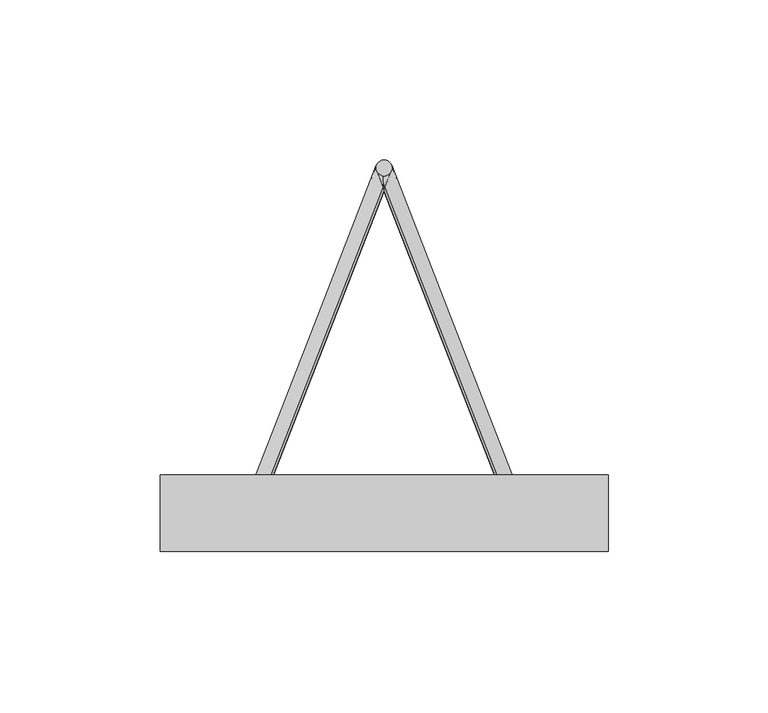
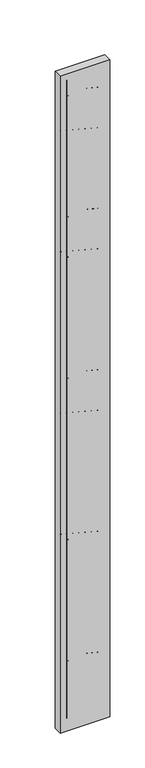
"""IFC4 building model written with IfcOpenShell, lengths in millimetres: proxy geometry, Vigota 1 (Pano 8) (Mf = 193)."""

from ifc_helpers import new_model, si_unit, point, frame, frame_2d, origin, origin_with_axes, origin_2d, place, context, project, spatial, polyline, circle_curve, trimmed, segment, composite_curve, outline, extrude, source, transform, mapped, element, save


def structural_framing_4a41f4d1(model_context):
    return source(origin(), model_context, "Body", "SweptSolid", [
        extrude(outline(polyline([(-70.0, 12.0), (70.0, 12.0), (70.0, -12.0), (-70.0, -12.0), (-70.0, 12.0)])), origin_with_axes(), (0.0, 0.0, 1.0), 1952.601886),
        extrude(outline(composite_curve([segment(trimmed(circle_curve(frame_2d((42.0, 0.0)), 2.5), [point((44.5, 0.0))], [point((39.5, 0.0))], False, "CARTESIAN"), True, "CONTINUOUS"), segment(trimmed(circle_curve(frame_2d((42.0, 0.0)), 2.5), [point((39.5, 0.0))], [point((44.5, 0.0))], False, "CARTESIAN"), True, "CONTINUOUS")], self_intersect=False)), frame((0.0, 0.0, 28.0), z_axis=(0.0, 0.0, 1.0), x_axis=(1.0, 0.0, 0.0)), (0.0, 0.0, 1.0), 1896.601886),
        extrude(outline(composite_curve([segment(trimmed(circle_curve(frame_2d((0.0, 108.0)), 2.5), [point((2.5, 108.0))], [point((-2.5, 108.0))], False, "CARTESIAN"), True, "CONTINUOUS"), segment(trimmed(circle_curve(frame_2d((0.0, 108.0)), 2.5), [point((-2.5, 108.0))], [point((2.5, 108.0))], False, "CARTESIAN"), True, "CONTINUOUS")], self_intersect=False)), frame((0.0, 0.0, 86.300943), z_axis=(0.0, 0.0, 1.0), x_axis=(1.0, 0.0, 0.0)), (0.0, 0.0, 1.0), 1780.0),
        extrude(outline(composite_curve([segment(trimmed(circle_curve(origin_2d(), 2.5), [point((2.5, 0.0))], [point((-2.5, 0.0))], False, "CARTESIAN"), True, "CONTINUOUS"), segment(trimmed(circle_curve(origin_2d(), 2.5), [point((-2.5, 0.0))], [point((2.5, 0.0))], False, "CARTESIAN"), True, "CONTINUOUS")], self_intersect=False)), frame((42.0, 0.0, 76.300943), z_axis=(-0.3218603428886276, 0.8276408817707567, 0.4598004898837537), x_axis=(0.8192319205108605, -3.936835275445103e-11, 0.5734623443750141)), (0.0, 0.0, 1.0), 130.491379),
        extrude(outline(composite_curve([segment(trimmed(circle_curve(origin_2d(), 2.5), [point((2.5, 0.0))], [point((-2.5, 0.0))], False, "CARTESIAN"), True, "CONTINUOUS"), segment(trimmed(circle_curve(origin_2d(), 2.5), [point((-2.5, 0.0))], [point((2.5, 0.0))], False, "CARTESIAN"), True, "CONTINUOUS")], self_intersect=False)), frame((0.0, 108.0, 136.300943), z_axis=(0.3218603428886276, -0.8276408817707567, 0.4598004898837537), x_axis=(0.8192319205108605, -3.936835275445103e-11, -0.5734623443750141)), (0.0, 0.0, 1.0), 130.491379),
        extrude(outline(composite_curve([segment(trimmed(circle_curve(origin_2d(), 2.5), [point((2.5, 0.0))], [point((-2.5, 0.0))], False, "CARTESIAN"), True, "CONTINUOUS"), segment(trimmed(circle_curve(origin_2d(), 2.5), [point((-2.5, 0.0))], [point((2.5, 0.0))], False, "CARTESIAN"), True, "CONTINUOUS")], self_intersect=False)), frame((42.0, 0.0, 196.300943), z_axis=(-0.3218603428886276, 0.8276408817707567, 0.4598004898837537), x_axis=(0.8192319205108605, -3.936835275445103e-11, 0.5734623443750141)), (0.0, 0.0, 1.0), 130.491379),
        extrude(outline(composite_curve([segment(trimmed(circle_curve(origin_2d(), 2.5), [point((2.5, 0.0))], [point((-2.5, 0.0))], False, "CARTESIAN"), True, "CONTINUOUS"), segment(trimmed(circle_curve(origin_2d(), 2.5), [point((-2.5, 0.0))], [point((2.5, 0.0))], False, "CARTESIAN"), True, "CONTINUOUS")], self_intersect=False)), frame((0.0, 108.0, 256.300943), z_axis=(0.3218603428886276, -0.8276408817707567, 0.4598004898837537), x_axis=(0.8192319205108605, -3.936835275445103e-11, -0.5734623443750141)), (0.0, 0.0, 1.0), 130.491379),
        extrude(outline(composite_curve([segment(trimmed(circle_curve(origin_2d(), 2.5), [point((2.5, 0.0))], [point((-2.5, 0.0))], False, "CARTESIAN"), True, "CONTINUOUS"), segment(trimmed(circle_curve(origin_2d(), 2.5), [point((-2.5, 0.0))], [point((2.5, 0.0))], False, "CARTESIAN"), True, "CONTINUOUS")], self_intersect=False)), frame((42.0, 0.0, 316.300943), z_axis=(-0.3218603428886276, 0.8276408817707567, 0.4598004898837537), x_axis=(0.8192319205108605, -3.936835275445103e-11, 0.5734623443750141)), (0.0, 0.0, 1.0), 130.491379),
        extrude(outline(composite_curve([segment(trimmed(circle_curve(origin_2d(), 2.5), [point((2.5, 0.0))], [point((-2.5, 0.0))], False, "CARTESIAN"), True, "CONTINUOUS"), segment(trimmed(circle_curve(origin_2d(), 2.5), [point((-2.5, 0.0))], [point((2.5, 0.0))], False, "CARTESIAN"), True, "CONTINUOUS")], self_intersect=False)), frame((0.0, 108.0, 376.300943), z_axis=(0.3218603428886276, -0.8276408817707567, 0.4598004898837537), x_axis=(0.8192319205108605, -3.936835275445103e-11, -0.5734623443750141)), (0.0, 0.0, 1.0), 130.491379),
        extrude(outline(composite_curve([segment(trimmed(circle_curve(origin_2d(), 2.5), [point((2.5, 0.0))], [point((-2.5, 0.0))], False, "CARTESIAN"), True, "CONTINUOUS"), segment(trimmed(circle_curve(origin_2d(), 2.5), [point((-2.5, 0.0))], [point((2.5, 0.0))], False, "CARTESIAN"), True, "CONTINUOUS")], self_intersect=False)), frame((42.0, 0.0, 436.300943), z_axis=(-0.3218603428886276, 0.8276408817707567, 0.4598004898837537), x_axis=(0.8192319205108605, -3.936835275445103e-11, 0.5734623443750141)), (0.0, 0.0, 1.0), 130.491379),
        extrude(outline(composite_curve([segment(trimmed(circle_curve(origin_2d(), 2.5), [point((2.5, 0.0))], [point((-2.5, 0.0))], False, "CARTESIAN"), True, "CONTINUOUS"), segment(trimmed(circle_curve(origin_2d(), 2.5), [point((-2.5, 0.0))], [point((2.5, 0.0))], False, "CARTESIAN"), True, "CONTINUOUS")], self_intersect=False)), frame((0.0, 108.0, 496.300943), z_axis=(0.3218603428886276, -0.8276408817707567, 0.4598004898837537), x_axis=(0.8192319205108605, -3.936835275445103e-11, -0.5734623443750141)), (0.0, 0.0, 1.0), 130.491379),
        extrude(outline(composite_curve([segment(trimmed(circle_curve(origin_2d(), 2.5), [point((2.5, 0.0))], [point((-2.5, 0.0))], False, "CARTESIAN"), True, "CONTINUOUS"), segment(trimmed(circle_curve(origin_2d(), 2.5), [point((-2.5, 0.0))], [point((2.5, 0.0))], False, "CARTESIAN"), True, "CONTINUOUS")], self_intersect=False)), frame((42.0, 0.0, 556.300943), z_axis=(-0.3218603428886276, 0.8276408817707567, 0.4598004898837537), x_axis=(0.8192319205108605, -3.936835275445103e-11, 0.5734623443750141)), (0.0, 0.0, 1.0), 130.491379),
        extrude(outline(composite_curve([segment(trimmed(circle_curve(origin_2d(), 2.5), [point((2.5, 0.0))], [point((-2.5, 0.0))], False, "CARTESIAN"), True, "CONTINUOUS"), segment(trimmed(circle_curve(origin_2d(), 2.5), [point((-2.5, 0.0))], [point((2.5, 0.0))], False, "CARTESIAN"), True, "CONTINUOUS")], self_intersect=False)), frame((0.0, 108.0, 616.300943), z_axis=(0.3218603428886276, -0.8276408817707567, 0.4598004898837537), x_axis=(0.8192319205108605, -3.936835275445103e-11, -0.5734623443750141)), (0.0, 0.0, 1.0), 130.491379),
        extrude(outline(composite_curve([segment(trimmed(circle_curve(origin_2d(), 2.5), [point((2.5, 0.0))], [point((-2.5, 0.0))], False, "CARTESIAN"), True, "CONTINUOUS"), segment(trimmed(circle_curve(origin_2d(), 2.5), [point((-2.5, 0.0))], [point((2.5, 0.0))], False, "CARTESIAN"), True, "CONTINUOUS")], self_intersect=False)), frame((42.0, 0.0, 676.300943), z_axis=(-0.3218603428886276, 0.8276408817707567, 0.4598004898837537), x_axis=(0.8192319205108605, -3.936835275445103e-11, 0.5734623443750141)), (0.0, 0.0, 1.0), 130.491379),
        extrude(outline(composite_curve([segment(trimmed(circle_curve(origin_2d(), 2.5), [point((2.5, 0.0))], [point((-2.5, 0.0))], False, "CARTESIAN"), True, "CONTINUOUS"), segment(trimmed(circle_curve(origin_2d(), 2.5), [point((-2.5, 0.0))], [point((2.5, 0.0))], False, "CARTESIAN"), True, "CONTINUOUS")], self_intersect=False)), frame((0.0, 108.0, 736.300943), z_axis=(0.3218603428886276, -0.8276408817707567, 0.4598004898837537), x_axis=(0.8192319205108605, -3.936835275445103e-11, -0.5734623443750141)), (0.0, 0.0, 1.0), 130.491379),
        extrude(outline(composite_curve([segment(trimmed(circle_curve(origin_2d(), 2.5), [point((2.5, 0.0))], [point((-2.5, 0.0))], False, "CARTESIAN"), True, "CONTINUOUS"), segment(trimmed(circle_curve(origin_2d(), 2.5), [point((-2.5, 0.0))], [point((2.5, 0.0))], False, "CARTESIAN"), True, "CONTINUOUS")], self_intersect=False)), frame((42.0, 0.0, 796.300943), z_axis=(-0.3218603428886276, 0.8276408817707567, 0.4598004898837537), x_axis=(0.8192319205108605, -3.936835275445103e-11, 0.5734623443750141)), (0.0, 0.0, 1.0), 130.491379),
        extrude(outline(composite_curve([segment(trimmed(circle_curve(origin_2d(), 2.5), [point((2.5, 0.0))], [point((-2.5, 0.0))], False, "CARTESIAN"), True, "CONTINUOUS"), segment(trimmed(circle_curve(origin_2d(), 2.5), [point((-2.5, 0.0))], [point((2.5, 0.0))], False, "CARTESIAN"), True, "CONTINUOUS")], self_intersect=False)), frame((0.0, 108.0, 856.300943), z_axis=(0.3218603428886276, -0.8276408817707567, 0.4598004898837537), x_axis=(0.8192319205108605, -3.936835275445103e-11, -0.5734623443750141)), (0.0, 0.0, 1.0), 130.491379),
        extrude(outline(composite_curve([segment(trimmed(circle_curve(origin_2d(), 2.5), [point((2.5, 0.0))], [point((-2.5, 0.0))], False, "CARTESIAN"), True, "CONTINUOUS"), segment(trimmed(circle_curve(origin_2d(), 2.5), [point((-2.5, 0.0))], [point((2.5, 0.0))], False, "CARTESIAN"), True, "CONTINUOUS")], self_intersect=False)), frame((42.0, 0.0, 916.300943), z_axis=(-0.3218603428886276, 0.8276408817707567, 0.4598004898837537), x_axis=(0.8192319205108605, -3.936835275445103e-11, 0.5734623443750141)), (0.0, 0.0, 1.0), 130.491379),
        extrude(outline(composite_curve([segment(trimmed(circle_curve(origin_2d(), 2.5), [point((2.5, 0.0))], [point((-2.5, 0.0))], False, "CARTESIAN"), True, "CONTINUOUS"), segment(trimmed(circle_curve(origin_2d(), 2.5), [point((-2.5, 0.0))], [point((2.5, 0.0))], False, "CARTESIAN"), True, "CONTINUOUS")], self_intersect=False)), frame((0.0, 108.0, 976.300943), z_axis=(0.3218603428886276, -0.8276408817707567, 0.4598004898837537), x_axis=(0.8192319205108605, -3.936835275445103e-11, -0.5734623443750141)), (0.0, 0.0, 1.0), 130.491379),
        extrude(outline(composite_curve([segment(trimmed(circle_curve(origin_2d(), 2.5), [point((2.5, 0.0))], [point((-2.5, 0.0))], False, "CARTESIAN"), True, "CONTINUOUS"), segment(trimmed(circle_curve(origin_2d(), 2.5), [point((-2.5, 0.0))], [point((2.5, 0.0))], False, "CARTESIAN"), True, "CONTINUOUS")], self_intersect=False)), frame((42.0, 0.0, 1036.300943), z_axis=(-0.3218603428886276, 0.8276408817707567, 0.4598004898837537), x_axis=(0.8192319205108605, -3.936835275445103e-11, 0.5734623443750141)), (0.0, 0.0, 1.0), 130.491379),
        extrude(outline(composite_curve([segment(trimmed(circle_curve(origin_2d(), 2.5), [point((2.5, 0.0))], [point((-2.5, 0.0))], False, "CARTESIAN"), True, "CONTINUOUS"), segment(trimmed(circle_curve(origin_2d(), 2.5), [point((-2.5, 0.0))], [point((2.5, 0.0))], False, "CARTESIAN"), True, "CONTINUOUS")], self_intersect=False)), frame((0.0, 108.0, 1096.300943), z_axis=(0.3218603428886276, -0.8276408817707567, 0.4598004898837537), x_axis=(0.8192319205108605, -3.936835275445103e-11, -0.5734623443750141)), (0.0, 0.0, 1.0), 130.491379),
        extrude(outline(composite_curve([segment(trimmed(circle_curve(origin_2d(), 2.5), [point((2.5, 0.0))], [point((-2.5, 0.0))], False, "CARTESIAN"), True, "CONTINUOUS"), segment(trimmed(circle_curve(origin_2d(), 2.5), [point((-2.5, 0.0))], [point((2.5, 0.0))], False, "CARTESIAN"), True, "CONTINUOUS")], self_intersect=False)), frame((42.0, 0.0, 1156.300943), z_axis=(-0.3218603428886276, 0.8276408817707567, 0.4598004898837537), x_axis=(0.8192319205108605, -3.936835275445103e-11, 0.5734623443750141)), (0.0, 0.0, 1.0), 130.491379),
        extrude(outline(composite_curve([segment(trimmed(circle_curve(origin_2d(), 2.5), [point((2.5, 0.0))], [point((-2.5, 0.0))], False, "CARTESIAN"), True, "CONTINUOUS"), segment(trimmed(circle_curve(origin_2d(), 2.5), [point((-2.5, 0.0))], [point((2.5, 0.0))], False, "CARTESIAN"), True, "CONTINUOUS")], self_intersect=False)), frame((0.0, 108.0, 1216.300943), z_axis=(0.3218603428886276, -0.8276408817707567, 0.4598004898837537), x_axis=(0.8192319205108605, -3.936835275445103e-11, -0.5734623443750141)), (0.0, 0.0, 1.0), 130.491379),
        extrude(outline(composite_curve([segment(trimmed(circle_curve(origin_2d(), 2.5), [point((2.5, 0.0))], [point((-2.5, 0.0))], False, "CARTESIAN"), True, "CONTINUOUS"), segment(trimmed(circle_curve(origin_2d(), 2.5), [point((-2.5, 0.0))], [point((2.5, 0.0))], False, "CARTESIAN"), True, "CONTINUOUS")], self_intersect=False)), frame((42.0, 0.0, 1276.300943), z_axis=(-0.3218603428886276, 0.8276408817707567, 0.4598004898837537), x_axis=(0.8192319205108605, -3.936835275445103e-11, 0.5734623443750141)), (0.0, 0.0, 1.0), 130.491379),
        extrude(outline(composite_curve([segment(trimmed(circle_curve(origin_2d(), 2.5), [point((2.5, 0.0))], [point((-2.5, 0.0))], False, "CARTESIAN"), True, "CONTINUOUS"), segment(trimmed(circle_curve(origin_2d(), 2.5), [point((-2.5, 0.0))], [point((2.5, 0.0))], False, "CARTESIAN"), True, "CONTINUOUS")], self_intersect=False)), frame((0.0, 108.0, 1336.300943), z_axis=(0.3218603428886276, -0.8276408817707567, 0.4598004898837537), x_axis=(0.8192319205108605, -3.936835275445103e-11, -0.5734623443750141)), (0.0, 0.0, 1.0), 130.491379),
        extrude(outline(composite_curve([segment(trimmed(circle_curve(origin_2d(), 2.5), [point((2.5, 0.0))], [point((-2.5, 0.0))], False, "CARTESIAN"), True, "CONTINUOUS"), segment(trimmed(circle_curve(origin_2d(), 2.5), [point((-2.5, 0.0))], [point((2.5, 0.0))], False, "CARTESIAN"), True, "CONTINUOUS")], self_intersect=False)), frame((42.0, 0.0, 1396.300943), z_axis=(-0.3218603428886276, 0.8276408817707567, 0.4598004898837537), x_axis=(0.8192319205108605, -3.936835275445103e-11, 0.5734623443750141)), (0.0, 0.0, 1.0), 130.491379),
        extrude(outline(composite_curve([segment(trimmed(circle_curve(origin_2d(), 2.5), [point((2.5, 0.0))], [point((-2.5, 0.0))], False, "CARTESIAN"), True, "CONTINUOUS"), segment(trimmed(circle_curve(origin_2d(), 2.5), [point((-2.5, 0.0))], [point((2.5, 0.0))], False, "CARTESIAN"), True, "CONTINUOUS")], self_intersect=False)), frame((0.0, 108.0, 1456.300943), z_axis=(0.3218603428886276, -0.8276408817707567, 0.4598004898837537), x_axis=(0.8192319205108605, -3.936835275445103e-11, -0.5734623443750141)), (0.0, 0.0, 1.0), 130.491379),
        extrude(outline(composite_curve([segment(trimmed(circle_curve(origin_2d(), 2.5), [point((2.5, 0.0))], [point((-2.5, 0.0))], False, "CARTESIAN"), True, "CONTINUOUS"), segment(trimmed(circle_curve(origin_2d(), 2.5), [point((-2.5, 0.0))], [point((2.5, 0.0))], False, "CARTESIAN"), True, "CONTINUOUS")], self_intersect=False)), frame((42.0, 0.0, 1516.300943), z_axis=(-0.3218603428886276, 0.8276408817707567, 0.4598004898837537), x_axis=(0.8192319205108605, -3.936835275445103e-11, 0.5734623443750141)), (0.0, 0.0, 1.0), 130.491379),
        extrude(outline(composite_curve([segment(trimmed(circle_curve(origin_2d(), 2.5), [point((2.5, 0.0))], [point((-2.5, 0.0))], False, "CARTESIAN"), True, "CONTINUOUS"), segment(trimmed(circle_curve(origin_2d(), 2.5), [point((-2.5, 0.0))], [point((2.5, 0.0))], False, "CARTESIAN"), True, "CONTINUOUS")], self_intersect=False)), frame((0.0, 108.0, 1576.300943), z_axis=(0.3218603428886276, -0.8276408817707567, 0.4598004898837537), x_axis=(0.8192319205108605, -3.936835275445103e-11, -0.5734623443750141)), (0.0, 0.0, 1.0), 130.491379),
        extrude(outline(composite_curve([segment(trimmed(circle_curve(origin_2d(), 2.5), [point((2.5, 0.0))], [point((-2.5, 0.0))], False, "CARTESIAN"), True, "CONTINUOUS"), segment(trimmed(circle_curve(origin_2d(), 2.5), [point((-2.5, 0.0))], [point((2.5, 0.0))], False, "CARTESIAN"), True, "CONTINUOUS")], self_intersect=False)), frame((42.0, 0.0, 1636.300943), z_axis=(-0.3218603428886276, 0.8276408817707567, 0.4598004898837537), x_axis=(0.8192319205108605, -3.936835275445103e-11, 0.5734623443750141)), (0.0, 0.0, 1.0), 130.491379),
        extrude(outline(composite_curve([segment(trimmed(circle_curve(origin_2d(), 2.5), [point((2.5, 0.0))], [point((-2.5, 0.0))], False, "CARTESIAN"), True, "CONTINUOUS"), segment(trimmed(circle_curve(origin_2d(), 2.5), [point((-2.5, 0.0))], [point((2.5, 0.0))], False, "CARTESIAN"), True, "CONTINUOUS")], self_intersect=False)), frame((0.0, 108.0, 1696.300943), z_axis=(0.3218603428886276, -0.8276408817707567, 0.4598004898837537), x_axis=(0.8192319205108605, -3.936835275445103e-11, -0.5734623443750141)), (0.0, 0.0, 1.0), 130.491379),
        extrude(outline(composite_curve([segment(trimmed(circle_curve(origin_2d(), 2.5), [point((2.5, 0.0))], [point((-2.5, 0.0))], False, "CARTESIAN"), True, "CONTINUOUS"), segment(trimmed(circle_curve(origin_2d(), 2.5), [point((-2.5, 0.0))], [point((2.5, 0.0))], False, "CARTESIAN"), True, "CONTINUOUS")], self_intersect=False)), frame((42.0, 0.0, 1756.300943), z_axis=(-0.3218603428886276, 0.8276408817707567, 0.4598004898837537), x_axis=(0.8192319205108605, -3.936835275445103e-11, 0.5734623443750141)), (0.0, 0.0, 1.0), 130.491379),
        extrude(outline(composite_curve([segment(trimmed(circle_curve(origin_2d(), 2.5), [point((2.5, 0.0))], [point((-2.5, 0.0))], False, "CARTESIAN"), True, "CONTINUOUS"), segment(trimmed(circle_curve(origin_2d(), 2.5), [point((-2.5, 0.0))], [point((2.5, 0.0))], False, "CARTESIAN"), True, "CONTINUOUS")], self_intersect=False)), frame((0.0, 108.0, 1816.300943), z_axis=(0.3218603428886276, -0.8276408817707567, 0.4598004898837537), x_axis=(0.8192319205108605, -3.936835275445103e-11, -0.5734623443750141)), (0.0, 0.0, 1.0), 130.491379),
        extrude(outline(composite_curve([segment(trimmed(circle_curve(frame_2d((-42.0, 0.0)), 2.5), [point((-39.5, 0.0))], [point((-44.5, 0.0))], False, "CARTESIAN"), True, "CONTINUOUS"), segment(trimmed(circle_curve(frame_2d((-42.0, 0.0)), 2.5), [point((-44.5, 0.0))], [point((-39.5, 0.0))], False, "CARTESIAN"), True, "CONTINUOUS")], self_intersect=False)), frame((0.0, 0.0, 28.0), z_axis=(0.0, 0.0, 1.0), x_axis=(1.0, 0.0, 0.0)), (0.0, 0.0, 1.0), 1896.601886),
        extrude(outline(composite_curve([segment(trimmed(circle_curve(origin_2d(), 2.5), [point((2.5, 0.0))], [point((-2.5, 0.0))], False, "CARTESIAN"), True, "CONTINUOUS"), segment(trimmed(circle_curve(origin_2d(), 2.5), [point((-2.5, 0.0))], [point((2.5, 0.0))], False, "CARTESIAN"), True, "CONTINUOUS")], self_intersect=False)), frame((-42.0, 0.0, 76.300943), z_axis=(0.3218603428886276, 0.8276408817707567, 0.4598004898837537), x_axis=(0.8192319205108605, 3.936835275445103e-11, -0.5734623443750141)), (0.0, 0.0, 1.0), 130.491379),
        extrude(outline(composite_curve([segment(trimmed(circle_curve(origin_2d(), 2.5), [point((2.5, 0.0))], [point((-2.5, 0.0))], False, "CARTESIAN"), True, "CONTINUOUS"), segment(trimmed(circle_curve(origin_2d(), 2.5), [point((-2.5, 0.0))], [point((2.5, 0.0))], False, "CARTESIAN"), True, "CONTINUOUS")], self_intersect=False)), frame((0.0, 108.0, 136.300943), z_axis=(-0.3218603428886276, -0.8276408817707567, 0.4598004898837537), x_axis=(0.8192319205108605, 3.936835275445103e-11, 0.5734623443750141)), (0.0, 0.0, 1.0), 130.491379),
        extrude(outline(composite_curve([segment(trimmed(circle_curve(origin_2d(), 2.5), [point((2.5, 0.0))], [point((-2.5, 0.0))], False, "CARTESIAN"), True, "CONTINUOUS"), segment(trimmed(circle_curve(origin_2d(), 2.5), [point((-2.5, 0.0))], [point((2.5, 0.0))], False, "CARTESIAN"), True, "CONTINUOUS")], self_intersect=False)), frame((-42.0, 0.0, 196.300943), z_axis=(0.3218603428886276, 0.8276408817707567, 0.4598004898837537), x_axis=(0.8192319205108605, 3.936835275445103e-11, -0.5734623443750141)), (0.0, 0.0, 1.0), 130.491379),
        extrude(outline(composite_curve([segment(trimmed(circle_curve(origin_2d(), 2.5), [point((2.5, 0.0))], [point((-2.5, 0.0))], False, "CARTESIAN"), True, "CONTINUOUS"), segment(trimmed(circle_curve(origin_2d(), 2.5), [point((-2.5, 0.0))], [point((2.5, 0.0))], False, "CARTESIAN"), True, "CONTINUOUS")], self_intersect=False)), frame((0.0, 108.0, 256.300943), z_axis=(-0.3218603428886276, -0.8276408817707567, 0.4598004898837537), x_axis=(0.8192319205108605, 3.936835275445103e-11, 0.5734623443750141)), (0.0, 0.0, 1.0), 130.491379),
        extrude(outline(composite_curve([segment(trimmed(circle_curve(origin_2d(), 2.5), [point((2.5, 0.0))], [point((-2.5, 0.0))], False, "CARTESIAN"), True, "CONTINUOUS"), segment(trimmed(circle_curve(origin_2d(), 2.5), [point((-2.5, 0.0))], [point((2.5, 0.0))], False, "CARTESIAN"), True, "CONTINUOUS")], self_intersect=False)), frame((-42.0, 0.0, 316.300943), z_axis=(0.3218603428886276, 0.8276408817707567, 0.4598004898837537), x_axis=(0.8192319205108605, 3.936835275445103e-11, -0.5734623443750141)), (0.0, 0.0, 1.0), 130.491379),
        extrude(outline(composite_curve([segment(trimmed(circle_curve(origin_2d(), 2.5), [point((2.5, 0.0))], [point((-2.5, 0.0))], False, "CARTESIAN"), True, "CONTINUOUS"), segment(trimmed(circle_curve(origin_2d(), 2.5), [point((-2.5, 0.0))], [point((2.5, 0.0))], False, "CARTESIAN"), True, "CONTINUOUS")], self_intersect=False)), frame((0.0, 108.0, 376.300943), z_axis=(-0.3218603428886276, -0.8276408817707567, 0.4598004898837537), x_axis=(0.8192319205108605, 3.936835275445103e-11, 0.5734623443750141)), (0.0, 0.0, 1.0), 130.491379),
        extrude(outline(composite_curve([segment(trimmed(circle_curve(origin_2d(), 2.5), [point((2.5, 0.0))], [point((-2.5, 0.0))], False, "CARTESIAN"), True, "CONTINUOUS"), segment(trimmed(circle_curve(origin_2d(), 2.5), [point((-2.5, 0.0))], [point((2.5, 0.0))], False, "CARTESIAN"), True, "CONTINUOUS")], self_intersect=False)), frame((-42.0, 0.0, 436.300943), z_axis=(0.3218603428886276, 0.8276408817707567, 0.4598004898837537), x_axis=(0.8192319205108605, 3.936835275445103e-11, -0.5734623443750141)), (0.0, 0.0, 1.0), 130.491379),
        extrude(outline(composite_curve([segment(trimmed(circle_curve(origin_2d(), 2.5), [point((2.5, 0.0))], [point((-2.5, 0.0))], False, "CARTESIAN"), True, "CONTINUOUS"), segment(trimmed(circle_curve(origin_2d(), 2.5), [point((-2.5, 0.0))], [point((2.5, 0.0))], False, "CARTESIAN"), True, "CONTINUOUS")], self_intersect=False)), frame((0.0, 108.0, 496.300943), z_axis=(-0.3218603428886276, -0.8276408817707567, 0.4598004898837537), x_axis=(0.8192319205108605, 3.936835275445103e-11, 0.5734623443750141)), (0.0, 0.0, 1.0), 130.491379),
        extrude(outline(composite_curve([segment(trimmed(circle_curve(origin_2d(), 2.5), [point((2.5, 0.0))], [point((-2.5, 0.0))], False, "CARTESIAN"), True, "CONTINUOUS"), segment(trimmed(circle_curve(origin_2d(), 2.5), [point((-2.5, 0.0))], [point((2.5, 0.0))], False, "CARTESIAN"), True, "CONTINUOUS")], self_intersect=False)), frame((-42.0, 0.0, 556.300943), z_axis=(0.3218603428886276, 0.8276408817707567, 0.4598004898837537), x_axis=(0.8192319205108605, 3.936835275445103e-11, -0.5734623443750141)), (0.0, 0.0, 1.0), 130.491379),
        extrude(outline(composite_curve([segment(trimmed(circle_curve(origin_2d(), 2.5), [point((2.5, 0.0))], [point((-2.5, 0.0))], False, "CARTESIAN"), True, "CONTINUOUS"), segment(trimmed(circle_curve(origin_2d(), 2.5), [point((-2.5, 0.0))], [point((2.5, 0.0))], False, "CARTESIAN"), True, "CONTINUOUS")], self_intersect=False)), frame((0.0, 108.0, 616.300943), z_axis=(-0.3218603428886276, -0.8276408817707567, 0.4598004898837537), x_axis=(0.8192319205108605, 3.936835275445103e-11, 0.5734623443750141)), (0.0, 0.0, 1.0), 130.491379),
        extrude(outline(composite_curve([segment(trimmed(circle_curve(origin_2d(), 2.5), [point((2.5, 0.0))], [point((-2.5, 0.0))], False, "CARTESIAN"), True, "CONTINUOUS"), segment(trimmed(circle_curve(origin_2d(), 2.5), [point((-2.5, 0.0))], [point((2.5, 0.0))], False, "CARTESIAN"), True, "CONTINUOUS")], self_intersect=False)), frame((-42.0, 0.0, 676.300943), z_axis=(0.3218603428886276, 0.8276408817707567, 0.4598004898837537), x_axis=(0.8192319205108605, 3.936835275445103e-11, -0.5734623443750141)), (0.0, 0.0, 1.0), 130.491379),
        extrude(outline(composite_curve([segment(trimmed(circle_curve(origin_2d(), 2.5), [point((2.5, 0.0))], [point((-2.5, 0.0))], False, "CARTESIAN"), True, "CONTINUOUS"), segment(trimmed(circle_curve(origin_2d(), 2.5), [point((-2.5, 0.0))], [point((2.5, 0.0))], False, "CARTESIAN"), True, "CONTINUOUS")], self_intersect=False)), frame((0.0, 108.0, 736.300943), z_axis=(-0.3218603428886276, -0.8276408817707567, 0.4598004898837537), x_axis=(0.8192319205108605, 3.936835275445103e-11, 0.5734623443750141)), (0.0, 0.0, 1.0), 130.491379),
        extrude(outline(composite_curve([segment(trimmed(circle_curve(origin_2d(), 2.5), [point((2.5, 0.0))], [point((-2.5, 0.0))], False, "CARTESIAN"), True, "CONTINUOUS"), segment(trimmed(circle_curve(origin_2d(), 2.5), [point((-2.5, 0.0))], [point((2.5, 0.0))], False, "CARTESIAN"), True, "CONTINUOUS")], self_intersect=False)), frame((-42.0, 0.0, 796.300943), z_axis=(0.3218603428886276, 0.8276408817707567, 0.4598004898837537), x_axis=(0.8192319205108605, 3.936835275445103e-11, -0.5734623443750141)), (0.0, 0.0, 1.0), 130.491379),
        extrude(outline(composite_curve([segment(trimmed(circle_curve(origin_2d(), 2.5), [point((2.5, 0.0))], [point((-2.5, 0.0))], False, "CARTESIAN"), True, "CONTINUOUS"), segment(trimmed(circle_curve(origin_2d(), 2.5), [point((-2.5, 0.0))], [point((2.5, 0.0))], False, "CARTESIAN"), True, "CONTINUOUS")], self_intersect=False)), frame((0.0, 108.0, 856.300943), z_axis=(-0.3218603428886276, -0.8276408817707567, 0.4598004898837537), x_axis=(0.8192319205108605, 3.936835275445103e-11, 0.5734623443750141)), (0.0, 0.0, 1.0), 130.491379),
        extrude(outline(composite_curve([segment(trimmed(circle_curve(origin_2d(), 2.5), [point((2.5, 0.0))], [point((-2.5, 0.0))], False, "CARTESIAN"), True, "CONTINUOUS"), segment(trimmed(circle_curve(origin_2d(), 2.5), [point((-2.5, 0.0))], [point((2.5, 0.0))], False, "CARTESIAN"), True, "CONTINUOUS")], self_intersect=False)), frame((-42.0, 0.0, 916.300943), z_axis=(0.3218603428886276, 0.8276408817707567, 0.4598004898837537), x_axis=(0.8192319205108605, 3.936835275445103e-11, -0.5734623443750141)), (0.0, 0.0, 1.0), 130.491379),
        extrude(outline(composite_curve([segment(trimmed(circle_curve(origin_2d(), 2.5), [point((2.5, 0.0))], [point((-2.5, 0.0))], False, "CARTESIAN"), True, "CONTINUOUS"), segment(trimmed(circle_curve(origin_2d(), 2.5), [point((-2.5, 0.0))], [point((2.5, 0.0))], False, "CARTESIAN"), True, "CONTINUOUS")], self_intersect=False)), frame((0.0, 108.0, 976.300943), z_axis=(-0.3218603428886276, -0.8276408817707567, 0.4598004898837537), x_axis=(0.8192319205108605, 3.936835275445103e-11, 0.5734623443750141)), (0.0, 0.0, 1.0), 130.491379),
        extrude(outline(composite_curve([segment(trimmed(circle_curve(origin_2d(), 2.5), [point((2.5, 0.0))], [point((-2.5, 0.0))], False, "CARTESIAN"), True, "CONTINUOUS"), segment(trimmed(circle_curve(origin_2d(), 2.5), [point((-2.5, 0.0))], [point((2.5, 0.0))], False, "CARTESIAN"), True, "CONTINUOUS")], self_intersect=False)), frame((-42.0, 0.0, 1036.300943), z_axis=(0.3218603428886276, 0.8276408817707567, 0.4598004898837537), x_axis=(0.8192319205108605, 3.936835275445103e-11, -0.5734623443750141)), (0.0, 0.0, 1.0), 130.491379),
        extrude(outline(composite_curve([segment(trimmed(circle_curve(origin_2d(), 2.5), [point((2.5, 0.0))], [point((-2.5, 0.0))], False, "CARTESIAN"), True, "CONTINUOUS"), segment(trimmed(circle_curve(origin_2d(), 2.5), [point((-2.5, 0.0))], [point((2.5, 0.0))], False, "CARTESIAN"), True, "CONTINUOUS")], self_intersect=False)), frame((0.0, 108.0, 1096.300943), z_axis=(-0.3218603428886276, -0.8276408817707567, 0.4598004898837537), x_axis=(0.8192319205108605, 3.936835275445103e-11, 0.5734623443750141)), (0.0, 0.0, 1.0), 130.491379),
        extrude(outline(composite_curve([segment(trimmed(circle_curve(origin_2d(), 2.5), [point((2.5, 0.0))], [point((-2.5, 0.0))], False, "CARTESIAN"), True, "CONTINUOUS"), segment(trimmed(circle_curve(origin_2d(), 2.5), [point((-2.5, 0.0))], [point((2.5, 0.0))], False, "CARTESIAN"), True, "CONTINUOUS")], self_intersect=False)), frame((-42.0, 0.0, 1156.300943), z_axis=(0.3218603428886276, 0.8276408817707567, 0.4598004898837537), x_axis=(0.8192319205108605, 3.936835275445103e-11, -0.5734623443750141)), (0.0, 0.0, 1.0), 130.491379),
        extrude(outline(composite_curve([segment(trimmed(circle_curve(origin_2d(), 2.5), [point((2.5, 0.0))], [point((-2.5, 0.0))], False, "CARTESIAN"), True, "CONTINUOUS"), segment(trimmed(circle_curve(origin_2d(), 2.5), [point((-2.5, 0.0))], [point((2.5, 0.0))], False, "CARTESIAN"), True, "CONTINUOUS")], self_intersect=False)), frame((0.0, 108.0, 1216.300943), z_axis=(-0.3218603428886276, -0.8276408817707567, 0.4598004898837537), x_axis=(0.8192319205108605, 3.936835275445103e-11, 0.5734623443750141)), (0.0, 0.0, 1.0), 130.491379),
        extrude(outline(composite_curve([segment(trimmed(circle_curve(origin_2d(), 2.5), [point((2.5, 0.0))], [point((-2.5, 0.0))], False, "CARTESIAN"), True, "CONTINUOUS"), segment(trimmed(circle_curve(origin_2d(), 2.5), [point((-2.5, 0.0))], [point((2.5, 0.0))], False, "CARTESIAN"), True, "CONTINUOUS")], self_intersect=False)), frame((-42.0, 0.0, 1276.300943), z_axis=(0.3218603428886276, 0.8276408817707567, 0.4598004898837537), x_axis=(0.8192319205108605, 3.936835275445103e-11, -0.5734623443750141)), (0.0, 0.0, 1.0), 130.491379),
        extrude(outline(composite_curve([segment(trimmed(circle_curve(origin_2d(), 2.5), [point((2.5, 0.0))], [point((-2.5, 0.0))], False, "CARTESIAN"), True, "CONTINUOUS"), segment(trimmed(circle_curve(origin_2d(), 2.5), [point((-2.5, 0.0))], [point((2.5, 0.0))], False, "CARTESIAN"), True, "CONTINUOUS")], self_intersect=False)), frame((0.0, 108.0, 1336.300943), z_axis=(-0.3218603428886276, -0.8276408817707567, 0.4598004898837537), x_axis=(0.8192319205108605, 3.936835275445103e-11, 0.5734623443750141)), (0.0, 0.0, 1.0), 130.491379),
        extrude(outline(composite_curve([segment(trimmed(circle_curve(origin_2d(), 2.5), [point((2.5, 0.0))], [point((-2.5, 0.0))], False, "CARTESIAN"), True, "CONTINUOUS"), segment(trimmed(circle_curve(origin_2d(), 2.5), [point((-2.5, 0.0))], [point((2.5, 0.0))], False, "CARTESIAN"), True, "CONTINUOUS")], self_intersect=False)), frame((-42.0, 0.0, 1396.300943), z_axis=(0.3218603428886276, 0.8276408817707567, 0.4598004898837537), x_axis=(0.8192319205108605, 3.936835275445103e-11, -0.5734623443750141)), (0.0, 0.0, 1.0), 130.491379),
        extrude(outline(composite_curve([segment(trimmed(circle_curve(origin_2d(), 2.5), [point((2.5, 0.0))], [point((-2.5, 0.0))], False, "CARTESIAN"), True, "CONTINUOUS"), segment(trimmed(circle_curve(origin_2d(), 2.5), [point((-2.5, 0.0))], [point((2.5, 0.0))], False, "CARTESIAN"), True, "CONTINUOUS")], self_intersect=False)), frame((0.0, 108.0, 1456.300943), z_axis=(-0.3218603428886276, -0.8276408817707567, 0.4598004898837537), x_axis=(0.8192319205108605, 3.936835275445103e-11, 0.5734623443750141)), (0.0, 0.0, 1.0), 130.491379),
        extrude(outline(composite_curve([segment(trimmed(circle_curve(origin_2d(), 2.5), [point((2.5, 0.0))], [point((-2.5, 0.0))], False, "CARTESIAN"), True, "CONTINUOUS"), segment(trimmed(circle_curve(origin_2d(), 2.5), [point((-2.5, 0.0))], [point((2.5, 0.0))], False, "CARTESIAN"), True, "CONTINUOUS")], self_intersect=False)), frame((-42.0, 0.0, 1516.300943), z_axis=(0.3218603428886276, 0.8276408817707567, 0.4598004898837537), x_axis=(0.8192319205108605, 3.936835275445103e-11, -0.5734623443750141)), (0.0, 0.0, 1.0), 130.491379),
        extrude(outline(composite_curve([segment(trimmed(circle_curve(origin_2d(), 2.5), [point((2.5, 0.0))], [point((-2.5, 0.0))], False, "CARTESIAN"), True, "CONTINUOUS"), segment(trimmed(circle_curve(origin_2d(), 2.5), [point((-2.5, 0.0))], [point((2.5, 0.0))], False, "CARTESIAN"), True, "CONTINUOUS")], self_intersect=False)), frame((0.0, 108.0, 1576.300943), z_axis=(-0.3218603428886276, -0.8276408817707567, 0.4598004898837537), x_axis=(0.8192319205108605, 3.936835275445103e-11, 0.5734623443750141)), (0.0, 0.0, 1.0), 130.491379),
        extrude(outline(composite_curve([segment(trimmed(circle_curve(origin_2d(), 2.5), [point((2.5, 0.0))], [point((-2.5, 0.0))], False, "CARTESIAN"), True, "CONTINUOUS"), segment(trimmed(circle_curve(origin_2d(), 2.5), [point((-2.5, 0.0))], [point((2.5, 0.0))], False, "CARTESIAN"), True, "CONTINUOUS")], self_intersect=False)), frame((-42.0, 0.0, 1636.300943), z_axis=(0.3218603428886276, 0.8276408817707567, 0.4598004898837537), x_axis=(0.8192319205108605, 3.936835275445103e-11, -0.5734623443750141)), (0.0, 0.0, 1.0), 130.491379),
        extrude(outline(composite_curve([segment(trimmed(circle_curve(origin_2d(), 2.5), [point((2.5, 0.0))], [point((-2.5, 0.0))], False, "CARTESIAN"), True, "CONTINUOUS"), segment(trimmed(circle_curve(origin_2d(), 2.5), [point((-2.5, 0.0))], [point((2.5, 0.0))], False, "CARTESIAN"), True, "CONTINUOUS")], self_intersect=False)), frame((0.0, 108.0, 1696.300943), z_axis=(-0.3218603428886276, -0.8276408817707567, 0.4598004898837537), x_axis=(0.8192319205108605, 3.936835275445103e-11, 0.5734623443750141)), (0.0, 0.0, 1.0), 130.491379),
        extrude(outline(composite_curve([segment(trimmed(circle_curve(origin_2d(), 2.5), [point((2.5, 0.0))], [point((-2.5, 0.0))], False, "CARTESIAN"), True, "CONTINUOUS"), segment(trimmed(circle_curve(origin_2d(), 2.5), [point((-2.5, 0.0))], [point((2.5, 0.0))], False, "CARTESIAN"), True, "CONTINUOUS")], self_intersect=False)), frame((-42.0, 0.0, 1756.300943), z_axis=(0.3218603428886276, 0.8276408817707567, 0.4598004898837537), x_axis=(0.8192319205108605, 3.936835275445103e-11, -0.5734623443750141)), (0.0, 0.0, 1.0), 130.491379),
        extrude(outline(composite_curve([segment(trimmed(circle_curve(origin_2d(), 2.5), [point((2.5, 0.0))], [point((-2.5, 0.0))], False, "CARTESIAN"), True, "CONTINUOUS"), segment(trimmed(circle_curve(origin_2d(), 2.5), [point((-2.5, 0.0))], [point((2.5, 0.0))], False, "CARTESIAN"), True, "CONTINUOUS")], self_intersect=False)), frame((0.0, 108.0, 1816.300943), z_axis=(-0.3218603428886276, -0.8276408817707567, 0.4598004898837537), x_axis=(0.8192319205108605, 3.936835275445103e-11, 0.5734623443750141)), (0.0, 0.0, 1.0), 130.491379),
    ])


if __name__ == "__main__":
    model = new_model("IFC4")
    model_context = context("Model", 3, world=origin())
    ifc_project = project(units=[si_unit("LENGTHUNIT", "METRE", prefix="MILLI")], contexts=[model_context])
    site = spatial("IfcSite", under=ifc_project)
    building = spatial("IfcBuilding", under=site)
    placement = place(None, origin())
    structural_framing_shape = structural_framing_4a41f4d1(model_context)
    element("IfcBuildingElementProxy", 1, Name="Vigota 1 (Pano 8) (Mf = 193)", ObjectType="Vigota 1 (Pano 8) (Mf = 193)", at=placement, inside=building, context=model_context, shape_type="MappedRepresentation", body=[
        mapped(structural_framing_shape, transform((0.0, 0.0, 0.0), x_axis=(1.0, 0.0, 0.0), y_axis=(0.0, 1.0, 0.0), z_axis=(0.0, 0.0, 1.0))),
    ])
    save(model, "model.ifc")

# Revit data of these elements
# Element 1 (IfcBuildingElementProxy, "Vigota 1 (Pano 8) (Mf = 193)")
#   Materials on its faces: "Aço", "Concreto armado"
# Materials
#   "Aço": class "Metal", colour RGB 120 120 120, transparency 0, Description = "Aço estrutural A36 grau, ASTM B, acabamento laminado", Cost = 0
#   "Concreto armado": class "Não atribuído", colour RGB 168 169 158, transparency 0
